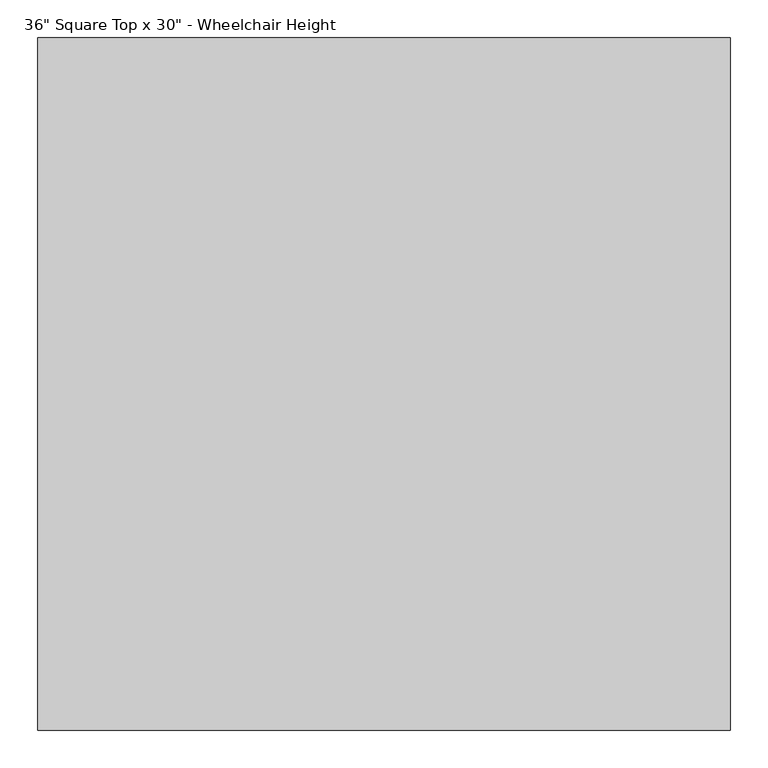
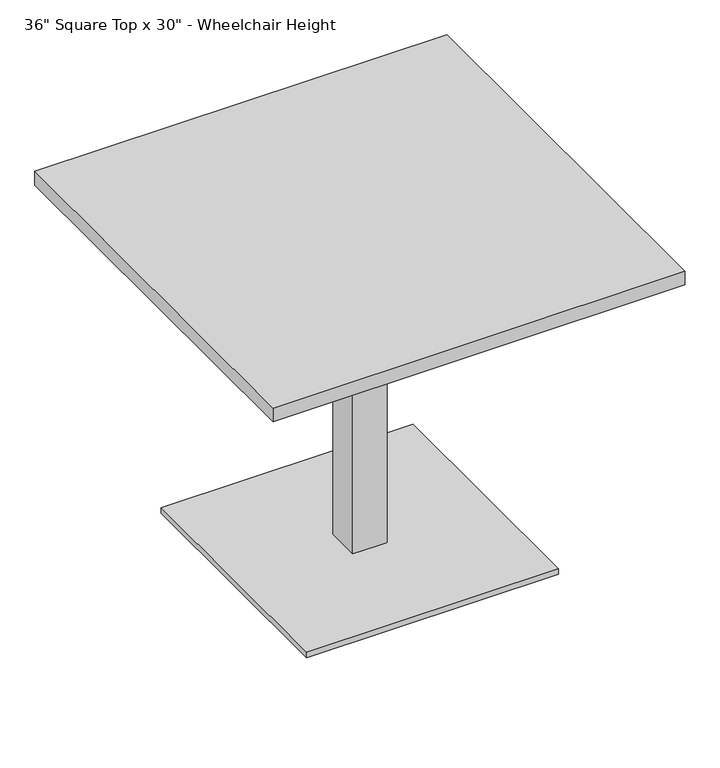
"""IFC4 building model written with IfcOpenShell, lengths in millimetres: furniture geometry."""

import ifcopenshell
import ifcopenshell.guid

model = None  # the IFC model being written
_history = None  # IfcOwnerHistory: only IFC2X3 demands one
_inside = {}  # id of a spatial element -> (the spatial element, [elements in it])
_under = {}  # id of a project, library or spatial element -> (it, [spatial elements below it])
_declared = {}  # id of a project -> (the project, [libraries it declares])
_typed = {}  # id of a type object -> (the type object, [elements of that type])
_made_of = {}  # id of a material, layer set ... -> (it, [elements and type objects made of it])


def new_model(schema):
    """Start an empty IFC model of exactly this schema.

    Asked for "IFC4X3", IfcOpenShell would pick the latest addendum, in which some entities
    have other attributes; the version numbers below select the first issue.
    IFC2X3 requires an IfcOwnerHistory on every rooted entity: one is made here for all.
    """
    global model, _history
    if schema == "IFC4X3":
        model = ifcopenshell.file(schema_version=(4, 3, 0, 0))
    else:
        model = ifcopenshell.file(schema=schema)
    _inside.clear()
    _under.clear()
    _declared.clear()
    _typed.clear()
    _made_of.clear()
    _history = None
    if model.schema == "IFC2X3":
        org = make("IfcOrganization", Name="unknown")
        user = make(
            "IfcPersonAndOrganization",
            ThePerson=make("IfcPerson", FamilyName="unknown"),
            TheOrganization=org,
        )
        app = make(
            "IfcApplication",
            ApplicationDeveloper=org,
            Version="unknown",
            ApplicationFullName="unknown",
            ApplicationIdentifier="unknown",
        )
        _history = make(
            "IfcOwnerHistory",
            OwningUser=user,
            OwningApplication=app,
            ChangeAction="ADDED",
            CreationDate=0,
        )
    return model


def make(cls, **values):
    """One entity of the class cls with the attributes given. An attribute that is None is left unset."""
    return model.create_entity(
        cls, **{name: value for name, value in values.items() if value is not None}
    )


def rooted(cls, **values):
    """An entity with a GlobalId (a new one), such as an element, a storey or a relation."""
    return make(cls, GlobalId=ifcopenshell.guid.new(), OwnerHistory=_history, **values)


def si_unit(unit_type, name, prefix=None):
    """IfcSIUnit, for example si_unit("LENGTHUNIT", "METRE", prefix="MILLI")."""
    return make("IfcSIUnit", UnitType=unit_type, Prefix=prefix, Name=name)


def assignment(units):
    """IfcUnitAssignment: the units of a project."""
    return None if units is None else make("IfcUnitAssignment", Units=units)


def point(xyz):
    """IfcCartesianPoint."""
    return None if xyz is None else make("IfcCartesianPoint", Coordinates=xyz)


def direction(xyz):
    """IfcDirection."""
    return None if xyz is None else make("IfcDirection", DirectionRatios=xyz)


def frame(location, z_axis=None, x_axis=None):
    """IfcAxis2Placement3D, a coordinate frame: its origin and axes. An axis left out is left unset."""
    return make(
        "IfcAxis2Placement3D",
        Location=point(location),
        Axis=direction(z_axis),
        RefDirection=direction(x_axis),
    )


def frame_2d(location, x_axis=None):
    """IfcAxis2Placement2D, a coordinate frame in the plane: its origin and x axis."""
    return make(
        "IfcAxis2Placement2D", Location=point(location), RefDirection=direction(x_axis)
    )


def origin():
    """The frame at (0, 0, 0) with its axes left unset."""
    return frame((0.0, 0.0, 0.0))


def origin_with_axes():
    """The frame at (0, 0, 0) with the z axis (0, 0, 1) and the x axis (1, 0, 0) written out."""
    return frame((0.0, 0.0, 0.0), z_axis=(0.0, 0.0, 1.0), x_axis=(1.0, 0.0, 0.0))


def place(relative_to, where):
    """IfcLocalPlacement: puts the frame where relative to a parent placement (None: the world)."""
    return make(
        "IfcLocalPlacement", PlacementRelTo=relative_to, RelativePlacement=where
    )


def context(
    kind, dimensions, precision=None, world=None, true_north=None, identifier=None
):
    """IfcGeometricRepresentationContext, for example the 3D "Model" context."""
    return make(
        "IfcGeometricRepresentationContext",
        ContextIdentifier=identifier,
        ContextType=kind,
        CoordinateSpaceDimension=dimensions,
        Precision=precision,
        WorldCoordinateSystem=world,
        TrueNorth=true_north,
    )


def project(units=None, contexts=None):
    """IfcProject with its units and contexts."""
    return rooted(
        "IfcProject",
        Name="project",
        RepresentationContexts=contexts,
        UnitsInContext=assignment(units),
    )


def spatial(cls, under=None, at=None, **own):
    """A site, building, storey or space (cls), placed at a placement, below another one or the project."""
    s = rooted(cls, ObjectPlacement=at, **own)
    if under is not None:
        _under.setdefault(under.id(), (under, []))[1].append(s)
    return s


def polyline(points):
    """IfcPolyline through the points."""
    return make("IfcPolyline", Points=[point(p) for p in points])


def circle_curve(where, radius):
    """IfcCircle in the frame where."""
    return make("IfcCircle", Position=where, Radius=radius)


def trimmed(basis, trim1, trim2, sense, master):
    """IfcTrimmedCurve: the piece of a basis curve between two trims."""
    return make(
        "IfcTrimmedCurve",
        BasisCurve=basis,
        Trim1=trim1,
        Trim2=trim2,
        SenseAgreement=sense,
        MasterRepresentation=master,
    )


def segment(curve, same_sense, transition):
    """IfcCompositeCurveSegment."""
    return make(
        "IfcCompositeCurveSegment",
        Transition=transition,
        SameSense=same_sense,
        ParentCurve=curve,
    )


def composite_curve(segments, self_intersect=None):
    """IfcCompositeCurve: segments joined end to end."""
    return make("IfcCompositeCurve", Segments=segments, SelfIntersect=self_intersect)


def outline(outer, holes=None, kind="AREA"):
    """IfcArbitraryClosedProfileDef: a profile drawn as a closed curve; with holes, ...WithVoids."""
    if holes is None:
        return make("IfcArbitraryClosedProfileDef", ProfileType=kind, OuterCurve=outer)
    return make(
        "IfcArbitraryProfileDefWithVoids",
        ProfileType=kind,
        OuterCurve=outer,
        InnerCurves=holes,
    )


def extrude(swept, where, along, depth):
    """IfcExtrudedAreaSolid: the profile swept, set in the frame where, extruded along a direction by depth."""
    return make(
        "IfcExtrudedAreaSolid",
        SweptArea=swept,
        Position=where,
        ExtrudedDirection=direction(along),
        Depth=depth,
    )


def shape(context_of_items, identifier, shape_type, items):
    """IfcShapeRepresentation: the items that make up one representation, for example the "Body"."""
    return make(
        "IfcShapeRepresentation",
        ContextOfItems=context_of_items,
        RepresentationIdentifier=identifier,
        RepresentationType=shape_type,
        Items=items,
    )


def source(mapping_origin, context_of_items, identifier, shape_type, items):
    """IfcRepresentationMap: a shape defined once, which mapped items show again and again."""
    return make(
        "IfcRepresentationMap",
        MappingOrigin=mapping_origin,
        MappedRepresentation=shape(context_of_items, identifier, shape_type, items),
    )


def transform(
    local_origin,
    x_axis=None,
    y_axis=None,
    z_axis=None,
    scale=None,
    scale2=None,
    scale3=None,
    uniform=True,
):
    """IfcCartesianTransformationOperator3D, or its non-uniform kind. x_axis, y_axis, z_axis: its Axis1, 2, 3."""
    if uniform:
        return make(
            "IfcCartesianTransformationOperator3D",
            Axis1=direction(x_axis),
            Axis2=direction(y_axis),
            LocalOrigin=point(local_origin),
            Scale=scale,
            Axis3=direction(z_axis),
        )
    return make(
        "IfcCartesianTransformationOperator3DnonUniform",
        Axis1=direction(x_axis),
        Axis2=direction(y_axis),
        LocalOrigin=point(local_origin),
        Scale=scale,
        Axis3=direction(z_axis),
        Scale2=scale2,
        Scale3=scale3,
    )


def mapped(mapping_source, mapping_target):
    """IfcMappedItem: shows the shape of a source again, moved by a transform."""
    return make(
        "IfcMappedItem", MappingSource=mapping_source, MappingTarget=mapping_target
    )


def made_of(thing, what):
    """Note that an element or type object is made of a material, layer set ...; save() writes the relation."""
    if what is not None:
        _made_of.setdefault(what.id(), (what, []))[1].append(thing)
    return thing


def element(
    cls,
    number,
    at=None,
    inside=None,
    cuts=None,
    type_object=None,
    material=None,
    context=None,
    identifier="Body",
    shape_type=None,
    held_by="IfcProductDefinitionShape",
    body=None,
    shapes=None,
    **own,
):
    """One element of the class cls, such as IfcWall. Its Tag is "e" and its number.

    at: its placement. inside: the storey or other place that contains it. cuts: it is an
    opening in that element (IfcRelVoidsElement). A single representation is given by context,
    identifier, shape_type and body (its items); several are given by shapes. held_by: the class
    of the entity that holds the representations. save() writes the other relations.
    """
    e = rooted(cls, Tag="e%d" % number, ObjectPlacement=at, **own)
    if body is not None:
        shapes = [shape(context, identifier, shape_type, body)]
    if shapes is not None:
        e.Representation = make(held_by, Representations=shapes)
    if inside is not None:
        _inside.setdefault(inside.id(), (inside, []))[1].append(e)
    if cuts is not None:
        rooted(
            "IfcRelVoidsElement", RelatingBuildingElement=cuts, RelatedOpeningElement=e
        )
    if type_object is not None:
        _typed.setdefault(type_object.id(), (type_object, []))[1].append(e)
    return made_of(e, material)


def aggregate(whole, parts):
    """IfcRelAggregates: a whole, such as a stair, and the parts it consists of."""
    return rooted("IfcRelAggregates", RelatingObject=whole, RelatedObjects=parts)


def save(model, path):
    """Write the relations noted so far, then the file.

    IfcRelAggregates (storeys below a building ...), IfcRelContainedInSpatialStructure (elements
    in a storey), IfcRelDefinesByType, IfcRelAssociatesMaterial and IfcRelDeclares: one each for
    every whole, place, type object, material and project.
    """
    for whole, parts in _under.values():
        aggregate(whole, parts)
    for where, things in _inside.values():
        rooted(
            "IfcRelContainedInSpatialStructure",
            RelatedElements=things,
            RelatingStructure=where,
        )
    for kind, things in _typed.values():
        rooted("IfcRelDefinesByType", RelatedObjects=things, RelatingType=kind)
    for what, things in _made_of.values():
        rooted("IfcRelAssociatesMaterial", RelatedObjects=things, RelatingMaterial=what)
    for by, libraries in _declared.values():
        rooted("IfcRelDeclares", RelatingContext=by, RelatedDefinitions=libraries)
    model.write(path)


def furniture_8b32ef4e(model_context):
    return source(origin(), model_context, "Body", "SweptSolid", [
        extrude(outline(composite_curve([segment(trimmed(circle_curve(frame_2d((107.7630735, 107.7630735)), 31.75), [point((77.0949285, 99.5455688))], [point((99.5455688, 77.0949285))], False, "CARTESIAN"), True, "CONTINUOUS"), segment(trimmed(circle_curve(frame_2d((97.9020678, 70.9612995)), 6.35), [point((99.5455688, 77.0949285))], [point((93.4119398, 75.4514275))], True, "CARTESIAN"), True, "CONTINUOUS"), segment(polyline([(93.4119398, 75.4514275), (17.9605122, 0.0), (93.4119398, -75.4514275)]), True, "CONTINUOUS"), segment(trimmed(circle_curve(frame_2d((97.9020678, -70.9612995)), 6.35), [point((93.4119398, -75.4514275))], [point((99.5455688, -77.0949285))], True, "CARTESIAN"), True, "CONTINUOUS"), segment(trimmed(circle_curve(frame_2d((107.7630735, -107.7630735)), 31.75), [point((99.5455688, -77.0949285))], [point((77.0949285, -99.5455688))], False, "CARTESIAN"), True, "CONTINUOUS"), segment(trimmed(circle_curve(frame_2d((70.9612995, -97.9020678)), 6.35), [point((77.0949285, -99.5455688))], [point((75.4514275, -93.4119398))], True, "CARTESIAN"), True, "CONTINUOUS"), segment(polyline([(75.4514275, -93.4119398), (0.0, -17.9605122), (-75.4514275, -93.4119398)]), True, "CONTINUOUS"), segment(trimmed(circle_curve(frame_2d((-70.9612995, -97.9020678)), 6.35), [point((-75.4514275, -93.4119398))], [point((-77.0949285, -99.5455688))], True, "CARTESIAN"), True, "CONTINUOUS"), segment(trimmed(circle_curve(frame_2d((-107.7630735, -107.7630735)), 31.75), [point((-77.0949285, -99.5455688))], [point((-99.5455688, -77.0949285))], False, "CARTESIAN"), True, "CONTINUOUS"), segment(trimmed(circle_curve(frame_2d((-97.9020678, -70.9612995)), 6.35), [point((-99.5455688, -77.0949285))], [point((-93.4119398, -75.4514275))], True, "CARTESIAN"), True, "CONTINUOUS"), segment(polyline([(-93.4119398, -75.4514275), (-17.9605122, 0.0), (-93.4119398, 75.4514275)]), True, "CONTINUOUS"), segment(trimmed(circle_curve(frame_2d((-97.9020678, 70.9612995)), 6.35), [point((-93.4119398, 75.4514275))], [point((-99.5455688, 77.0949285))], True, "CARTESIAN"), True, "CONTINUOUS"), segment(trimmed(circle_curve(frame_2d((-107.7630735, 107.7630735)), 31.75), [point((-99.5455688, 77.0949285))], [point((-77.0949285, 99.5455688))], False, "CARTESIAN"), True, "CONTINUOUS"), segment(trimmed(circle_curve(frame_2d((-70.9612995, 97.9020678)), 6.35), [point((-77.0949285, 99.5455688))], [point((-75.4514275, 93.4119398))], True, "CARTESIAN"), True, "CONTINUOUS"), segment(polyline([(-75.4514275, 93.4119398), (0.0, 17.9605122), (75.4514275, 93.4119398)]), True, "CONTINUOUS"), segment(trimmed(circle_curve(frame_2d((70.9612995, 97.9020678)), 6.35), [point((75.4514275, 93.4119398))], [point((77.0949285, 99.5455688))], True, "CARTESIAN"), True, "CONTINUOUS")], self_intersect=False)), frame((0.0, 0.0, 723.9), z_axis=(0.0, 0.0, 1.0), x_axis=(1.0, 0.0, 0.0)), (0.0, 0.0, 1.0), 6.35),
        extrude(outline(polyline([(-38.1, 38.1), (38.1, 38.1), (38.1, -38.1), (-38.1, -38.1), (-38.1, 38.1)])), frame((0.0, 0.0, 19.05), z_axis=(0.0, 0.0, 1.0), x_axis=(1.0, 0.0, 0.0)), (0.0, 0.0, 1.0), 704.85),
        extrude(outline(composite_curve([segment(trimmed(circle_curve(frame_2d((-251.0506403, -251.0506403)), 12.7), [point((-263.7506403, -251.0506403))], [point((-238.3506403, -251.0506403))], False, "CARTESIAN"), True, "CONTINUOUS"), segment(trimmed(circle_curve(frame_2d((-251.0506403, -251.0506403)), 12.7), [point((-238.3506403, -251.0506403))], [point((-263.7506403, -251.0506403))], False, "CARTESIAN"), True, "CONTINUOUS")], self_intersect=False)), origin_with_axes(), (0.0, 0.0, 1.0), 6.35),
        extrude(outline(composite_curve([segment(trimmed(circle_curve(frame_2d((-251.0506403, 251.0506403)), 12.7), [point((-263.7506403, 251.0506403))], [point((-238.3506403, 251.0506403))], False, "CARTESIAN"), True, "CONTINUOUS"), segment(trimmed(circle_curve(frame_2d((-251.0506403, 251.0506403)), 12.7), [point((-238.3506403, 251.0506403))], [point((-263.7506403, 251.0506403))], False, "CARTESIAN"), True, "CONTINUOUS")], self_intersect=False)), origin_with_axes(), (0.0, 0.0, 1.0), 6.35),
        extrude(outline(composite_curve([segment(trimmed(circle_curve(frame_2d((251.0506403, -251.0506403)), 12.7), [point((238.3506403, -251.0506403))], [point((263.7506403, -251.0506403))], False, "CARTESIAN"), True, "CONTINUOUS"), segment(trimmed(circle_curve(frame_2d((251.0506403, -251.0506403)), 12.7), [point((263.7506403, -251.0506403))], [point((238.3506403, -251.0506403))], False, "CARTESIAN"), True, "CONTINUOUS")], self_intersect=False)), origin_with_axes(), (0.0, 0.0, 1.0), 6.35),
        extrude(outline(composite_curve([segment(trimmed(circle_curve(frame_2d((251.0506403, 251.0506403)), 12.7), [point((238.3506403, 251.0506403))], [point((263.7506403, 251.0506403))], False, "CARTESIAN"), True, "CONTINUOUS"), segment(trimmed(circle_curve(frame_2d((251.0506403, 251.0506403)), 12.7), [point((263.7506403, 251.0506403))], [point((238.3506403, 251.0506403))], False, "CARTESIAN"), True, "CONTINUOUS")], self_intersect=False)), origin_with_axes(), (0.0, 0.0, 1.0), 6.35),
        extrude(outline(polyline([(279.4, 279.4), (279.4, -279.4), (-279.4, -279.4), (-279.4, 279.4), (279.4, 279.4)])), frame((0.0, 0.0, 6.35), z_axis=(0.0, 0.0, 1.0), x_axis=(1.0, 0.0, 0.0)), (0.0, 0.0, 1.0), 12.7),
        extrude(outline(polyline([(457.2, 457.2), (457.2, -457.2), (-457.2, -457.2), (-457.2, 457.2), (457.2, 457.2)])), frame((0.0, 0.0, 730.25), z_axis=(0.0, 0.0, 1.0), x_axis=(1.0, 0.0, 0.0)), (0.0, 0.0, 1.0), 31.75),
    ])


if __name__ == "__main__":
    model = new_model("IFC4")
    model_context = context("Model", 3, world=origin())
    ifc_project = project(units=[si_unit("LENGTHUNIT", "METRE", prefix="MILLI")], contexts=[model_context])
    site = spatial("IfcSite", under=ifc_project)
    building = spatial("IfcBuilding", under=site)
    placement = place(None, origin())
    furniture_shape = furniture_8b32ef4e(model_context)
    element("IfcFurniture", 1, ObjectType="Falcon 7700 Series Pedestal Base : 36\" Square Top x 30\" - Wheelchair Height", at=placement, inside=building, context=model_context, shape_type="MappedRepresentation", body=[
        mapped(furniture_shape, transform((0.0, 0.0, 0.0), x_axis=(1.0, 0.0, 0.0), y_axis=(0.0, 1.0, 0.0), z_axis=(0.0, 0.0, 1.0))),
    ])
    save(model, "model.ifc")

# Revit data of these elements
# Type "Falcon 7700 Series Pedestal Base : 36\" Square Top x 30\" - Wheelchair Height"
#   URL = "http://www.commercialfurnituregroup.com/"
#   Product URL = "http://www.falconproducts.com/product/10525/Square-Table-Base.html"
#   Modeled By [instance default] = "http://www.therevitcollection.com"
#   Model Line = "Table Bases"
#   Model = "7700 Series"
#   Description = "Single Pedestal Table Base"
#   Brand = "Falcon"
#   Manufacturer = "Commercial Furniture Group Inc."
#   Assembly Code = "E2020200"
#   Table Width = 3' - 0"
#   Table Depth = 3' - 0"
#   Radius = 1' - 6"
#   Base Width = 1' - 10"
#   Table Thickness [instance default] = 0' - 1 1/4"
#   Height = 2' - 6"
#   Base Depth = 1' - 10"
#   Roundtop = no
#   RectangleTop = yes
#   Tabletop [instance default] = none
#   Table Base [instance default] = none
#   Type Comments = ""
#   Default Elevation = 0
# Element 1 (IfcFurniture, "Falcon 7700 Series Pedestal Base : 36\" Square Top x 30\" - Wheelchair Height")
#   Tabletop = Metal - Aluminum
#   Table Base = Metal - Aluminum
#   Materials on its faces: "Metal - Aluminum"
# Materials
#   "Metal - Aluminum": class "Metal", colour RGB 247 247 247, transparency 0
